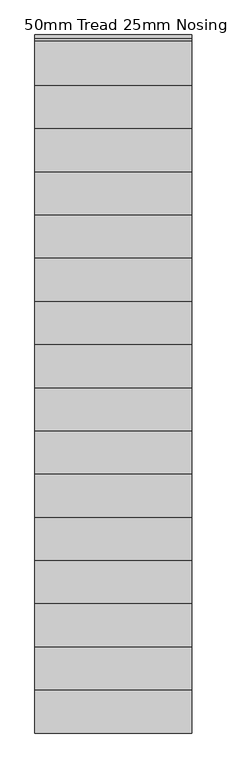
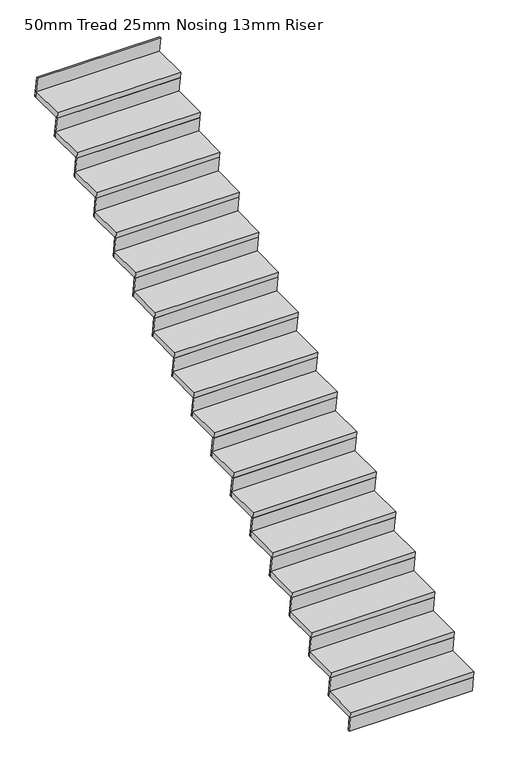
"""IFC4 building model written with IfcOpenShell, lengths in millimetres: stair flight geometry, 50mm Tread 25mm Nosing 13mm Riser."""

from ifc_helpers import new_model, si_unit, frame, origin, place, context, project, spatial, polyline, outline, extrude, source, transform, mapped, element, save


def stair_flight_50mm_tread_25mm_nosing_13mm_riser_8afb8e9e(model_context):
    return source(origin(), model_context, "Body", "SweptSolid", [
        extrude(outline(polyline([(-30533.3785178, 176.4705882), (-30233.3785178, 176.4705882), (-30226.2951845, 126.4705882), (-30526.2951845, 126.4705882), (-30533.3785178, 176.4705882)])), frame((125666.3174172, 0.0, 0.0), z_axis=(1.0, 0.0, 0.0), x_axis=(0.0, 1.0, 0.0)), (0.0, 0.0, 1.0), 1000.0),
        extrude(outline(polyline([(-30526.2951845, 126.4705882), (-30513.6703736, 126.4705882), (-30495.7537069, 0.0), (-30508.3785178, 0.0), (-30526.2951845, 126.4705882)])), frame((125666.3174172, 0.0, 0.0), z_axis=(1.0, 0.0, 0.0), x_axis=(0.0, 1.0, 0.0)), (0.0, 0.0, 1.0), 1000.0),
        extrude(outline(polyline([(-30251.2951845, 302.9411765), (-30238.6703736, 302.9411765), (-30213.6703736, 126.4705882), (-30226.2951845, 126.4705882), (-30251.2951845, 302.9411765)])), frame((125666.3174172, 0.0, 0.0), z_axis=(1.0, 0.0, 0.0), x_axis=(0.0, 1.0, 0.0)), (0.0, 0.0, 1.0), 1000.0),
        extrude(outline(polyline([(-30258.3785178, 352.9411765), (-29958.3785178, 352.9411765), (-29951.2951845, 302.9411765), (-30251.2951845, 302.9411765), (-30258.3785178, 352.9411765)])), frame((125666.3174172, 0.0, 0.0), z_axis=(1.0, 0.0, 0.0), x_axis=(0.0, 1.0, 0.0)), (0.0, 0.0, 1.0), 1000.0),
        extrude(outline(polyline([(-29976.2951845, 479.4117647), (-29963.6703736, 479.4117647), (-29938.6703736, 302.9411765), (-29951.2951845, 302.9411765), (-29976.2951845, 479.4117647)])), frame((125666.3174172, 0.0, 0.0), z_axis=(1.0, 0.0, 0.0), x_axis=(0.0, 1.0, 0.0)), (0.0, 0.0, 1.0), 1000.0),
        extrude(outline(polyline([(-29983.3785178, 529.4117647), (-29683.3785178, 529.4117647), (-29676.2951845, 479.4117647), (-29976.2951845, 479.4117647), (-29983.3785178, 529.4117647)])), frame((125666.3174172, 0.0, 0.0), z_axis=(1.0, 0.0, 0.0), x_axis=(0.0, 1.0, 0.0)), (0.0, 0.0, 1.0), 1000.0),
        extrude(outline(polyline([(-29701.2951845, 655.8823529), (-29688.6703736, 655.8823529), (-29663.6703736, 479.4117647), (-29676.2951845, 479.4117647), (-29701.2951845, 655.8823529)])), frame((125666.3174172, 0.0, 0.0), z_axis=(1.0, 0.0, 0.0), x_axis=(0.0, 1.0, 0.0)), (0.0, 0.0, 1.0), 1000.0),
        extrude(outline(polyline([(-29708.3785178, 705.8823529), (-29408.3785178, 705.8823529), (-29401.2951845, 655.8823529), (-29701.2951845, 655.8823529), (-29708.3785178, 705.8823529)])), frame((125666.3174172, 0.0, 0.0), z_axis=(1.0, 0.0, 0.0), x_axis=(0.0, 1.0, 0.0)), (0.0, 0.0, 1.0), 1000.0),
        extrude(outline(polyline([(-29426.2951845, 832.3529412), (-29413.6703736, 832.3529412), (-29388.6703736, 655.8823529), (-29401.2951845, 655.8823529), (-29426.2951845, 832.3529412)])), frame((125666.3174172, 0.0, 0.0), z_axis=(1.0, 0.0, 0.0), x_axis=(0.0, 1.0, 0.0)), (0.0, 0.0, 1.0), 1000.0),
        extrude(outline(polyline([(-29433.3785178, 882.3529412), (-29133.3785178, 882.3529412), (-29126.2951845, 832.3529412), (-29426.2951845, 832.3529412), (-29433.3785178, 882.3529412)])), frame((125666.3174172, 0.0, 0.0), z_axis=(1.0, 0.0, 0.0), x_axis=(0.0, 1.0, 0.0)), (0.0, 0.0, 1.0), 1000.0),
        extrude(outline(polyline([(-29151.2951845, 1008.8235294), (-29138.6703736, 1008.8235294), (-29113.6703736, 832.3529412), (-29126.2951845, 832.3529412), (-29151.2951845, 1008.8235294)])), frame((125666.3174172, 0.0, 0.0), z_axis=(1.0, 0.0, 0.0), x_axis=(0.0, 1.0, 0.0)), (0.0, 0.0, 1.0), 1000.0),
        extrude(outline(polyline([(-29158.3785178, 1058.8235294), (-28858.3785178, 1058.8235294), (-28851.2951845, 1008.8235294), (-29151.2951845, 1008.8235294), (-29158.3785178, 1058.8235294)])), frame((125666.3174172, 0.0, 0.0), z_axis=(1.0, 0.0, 0.0), x_axis=(0.0, 1.0, 0.0)), (0.0, 0.0, 1.0), 1000.0),
        extrude(outline(polyline([(-28876.2951845, 1185.2941176), (-28863.6703736, 1185.2941176), (-28838.6703736, 1008.8235294), (-28851.2951845, 1008.8235294), (-28876.2951845, 1185.2941176)])), frame((125666.3174172, 0.0, 0.0), z_axis=(1.0, 0.0, 0.0), x_axis=(0.0, 1.0, 0.0)), (0.0, 0.0, 1.0), 1000.0),
        extrude(outline(polyline([(-28883.3785178, 1235.2941176), (-28583.3785178, 1235.2941176), (-28576.2951845, 1185.2941176), (-28876.2951845, 1185.2941176), (-28883.3785178, 1235.2941176)])), frame((125666.3174172, 0.0, 0.0), z_axis=(1.0, 0.0, 0.0), x_axis=(0.0, 1.0, 0.0)), (0.0, 0.0, 1.0), 1000.0),
        extrude(outline(polyline([(-28601.2951845, 1361.7647059), (-28588.6703736, 1361.7647059), (-28563.6703736, 1185.2941176), (-28576.2951845, 1185.2941176), (-28601.2951845, 1361.7647059)])), frame((125666.3174172, 0.0, 0.0), z_axis=(1.0, 0.0, 0.0), x_axis=(0.0, 1.0, 0.0)), (0.0, 0.0, 1.0), 1000.0),
        extrude(outline(polyline([(-28608.3785178, 1411.7647059), (-28308.3785178, 1411.7647059), (-28301.2951845, 1361.7647059), (-28601.2951845, 1361.7647059), (-28608.3785178, 1411.7647059)])), frame((125666.3174172, 0.0, 0.0), z_axis=(1.0, 0.0, 0.0), x_axis=(0.0, 1.0, 0.0)), (0.0, 0.0, 1.0), 1000.0),
        extrude(outline(polyline([(-28326.2951845, 1538.2352941), (-28313.6703736, 1538.2352941), (-28288.6703736, 1361.7647059), (-28301.2951845, 1361.7647059), (-28326.2951845, 1538.2352941)])), frame((125666.3174172, 0.0, 0.0), z_axis=(1.0, 0.0, 0.0), x_axis=(0.0, 1.0, 0.0)), (0.0, 0.0, 1.0), 1000.0),
        extrude(outline(polyline([(-28333.3785178, 1588.2352941), (-28033.3785178, 1588.2352941), (-28026.2951845, 1538.2352941), (-28326.2951845, 1538.2352941), (-28333.3785178, 1588.2352941)])), frame((125666.3174172, 0.0, 0.0), z_axis=(1.0, 0.0, 0.0), x_axis=(0.0, 1.0, 0.0)), (0.0, 0.0, 1.0), 1000.0),
        extrude(outline(polyline([(-28051.2951845, 1714.7058824), (-28038.6703736, 1714.7058824), (-28013.6703736, 1538.2352941), (-28026.2951845, 1538.2352941), (-28051.2951845, 1714.7058824)])), frame((125666.3174172, 0.0, 0.0), z_axis=(1.0, 0.0, 0.0), x_axis=(0.0, 1.0, 0.0)), (0.0, 0.0, 1.0), 1000.0),
        extrude(outline(polyline([(-28058.3785178, 1764.7058824), (-27758.3785178, 1764.7058824), (-27751.2951845, 1714.7058824), (-28051.2951845, 1714.7058824), (-28058.3785178, 1764.7058824)])), frame((125666.3174172, 0.0, 0.0), z_axis=(1.0, 0.0, 0.0), x_axis=(0.0, 1.0, 0.0)), (0.0, 0.0, 1.0), 1000.0),
        extrude(outline(polyline([(-27776.2951845, 1891.1764706), (-27763.6703736, 1891.1764706), (-27738.6703736, 1714.7058824), (-27751.2951845, 1714.7058824), (-27776.2951845, 1891.1764706)])), frame((125666.3174172, 0.0, 0.0), z_axis=(1.0, 0.0, 0.0), x_axis=(0.0, 1.0, 0.0)), (0.0, 0.0, 1.0), 1000.0),
        extrude(outline(polyline([(-27783.3785178, 1941.1764706), (-27483.3785178, 1941.1764706), (-27476.2951845, 1891.1764706), (-27776.2951845, 1891.1764706), (-27783.3785178, 1941.1764706)])), frame((125666.3174172, 0.0, 0.0), z_axis=(1.0, 0.0, 0.0), x_axis=(0.0, 1.0, 0.0)), (0.0, 0.0, 1.0), 1000.0),
        extrude(outline(polyline([(-27501.2951845, 2067.6470588), (-27488.6703736, 2067.6470588), (-27463.6703736, 1891.1764706), (-27476.2951845, 1891.1764706), (-27501.2951845, 2067.6470588)])), frame((125666.3174172, 0.0, 0.0), z_axis=(1.0, 0.0, 0.0), x_axis=(0.0, 1.0, 0.0)), (0.0, 0.0, 1.0), 1000.0),
        extrude(outline(polyline([(-27508.3785178, 2117.6470588), (-27208.3785178, 2117.6470588), (-27201.2951845, 2067.6470588), (-27501.2951845, 2067.6470588), (-27508.3785178, 2117.6470588)])), frame((125666.3174172, 0.0, 0.0), z_axis=(1.0, 0.0, 0.0), x_axis=(0.0, 1.0, 0.0)), (0.0, 0.0, 1.0), 1000.0),
        extrude(outline(polyline([(-27226.2951845, 2244.1176471), (-27213.6703736, 2244.1176471), (-27188.6703736, 2067.6470588), (-27201.2951845, 2067.6470588), (-27226.2951845, 2244.1176471)])), frame((125666.3174172, 0.0, 0.0), z_axis=(1.0, 0.0, 0.0), x_axis=(0.0, 1.0, 0.0)), (0.0, 0.0, 1.0), 1000.0),
        extrude(outline(polyline([(-27233.3785178, 2294.1176471), (-26933.3785178, 2294.1176471), (-26926.2951845, 2244.1176471), (-27226.2951845, 2244.1176471), (-27233.3785178, 2294.1176471)])), frame((125666.3174172, 0.0, 0.0), z_axis=(1.0, 0.0, 0.0), x_axis=(0.0, 1.0, 0.0)), (0.0, 0.0, 1.0), 1000.0),
        extrude(outline(polyline([(-26951.2951845, 2420.5882353), (-26938.6703736, 2420.5882353), (-26913.6703736, 2244.1176471), (-26926.2951845, 2244.1176471), (-26951.2951845, 2420.5882353)])), frame((125666.3174172, 0.0, 0.0), z_axis=(1.0, 0.0, 0.0), x_axis=(0.0, 1.0, 0.0)), (0.0, 0.0, 1.0), 1000.0),
        extrude(outline(polyline([(-26958.3785178, 2470.5882353), (-26658.3785178, 2470.5882353), (-26651.2951845, 2420.5882353), (-26951.2951845, 2420.5882353), (-26958.3785178, 2470.5882353)])), frame((125666.3174172, 0.0, 0.0), z_axis=(1.0, 0.0, 0.0), x_axis=(0.0, 1.0, 0.0)), (0.0, 0.0, 1.0), 1000.0),
        extrude(outline(polyline([(-26676.2951845, 2597.0588235), (-26663.6703736, 2597.0588235), (-26638.6703736, 2420.5882353), (-26651.2951845, 2420.5882353), (-26676.2951845, 2597.0588235)])), frame((125666.3174172, 0.0, 0.0), z_axis=(1.0, 0.0, 0.0), x_axis=(0.0, 1.0, 0.0)), (0.0, 0.0, 1.0), 1000.0),
        extrude(outline(polyline([(-26683.3785178, 2647.0588235), (-26383.3785178, 2647.0588235), (-26376.2951845, 2597.0588235), (-26676.2951845, 2597.0588235), (-26683.3785178, 2647.0588235)])), frame((125666.3174172, 0.0, 0.0), z_axis=(1.0, 0.0, 0.0), x_axis=(0.0, 1.0, 0.0)), (0.0, 0.0, 1.0), 1000.0),
        extrude(outline(polyline([(-26401.2951845, 2773.5294118), (-26388.6703736, 2773.5294118), (-26363.6703736, 2597.0588235), (-26376.2951845, 2597.0588235), (-26401.2951845, 2773.5294118)])), frame((125666.3174172, 0.0, 0.0), z_axis=(1.0, 0.0, 0.0), x_axis=(0.0, 1.0, 0.0)), (0.0, 0.0, 1.0), 1000.0),
        extrude(outline(polyline([(-26126.2951845, 2950.0), (-26113.6703736, 2950.0), (-26088.6703736, 2773.5294118), (-26101.2951845, 2773.5294118), (-26126.2951845, 2950.0)])), frame((125666.3174172, 0.0, 0.0), z_axis=(1.0, 0.0, 0.0), x_axis=(0.0, 1.0, 0.0)), (0.0, 0.0, 1.0), 1000.0),
        extrude(outline(polyline([(-26408.3785178, 2823.5294118), (-26108.3785178, 2823.5294118), (-26101.2951845, 2773.5294118), (-26401.2951845, 2773.5294118), (-26408.3785178, 2823.5294118)])), frame((125666.3174172, 0.0, 0.0), z_axis=(1.0, 0.0, 0.0), x_axis=(0.0, 1.0, 0.0)), (0.0, 0.0, 1.0), 1000.0),
    ])


if __name__ == "__main__":
    model = new_model("IFC4")
    model_context = context("Model", 3, world=origin())
    ifc_project = project(units=[si_unit("LENGTHUNIT", "METRE", prefix="MILLI")], contexts=[model_context])
    site = spatial("IfcSite", under=ifc_project)
    building = spatial("IfcBuilding", under=site)
    placement = place(None, origin())
    stair_flight_50mm_tread_25mm_nosing_13mm_riser_shape = stair_flight_50mm_tread_25mm_nosing_13mm_riser_8afb8e9e(model_context)
    element("IfcStairFlight", 1, ObjectType="50mm Tread 25mm Nosing 13mm Riser", at=placement, inside=building, context=model_context, shape_type="MappedRepresentation", body=[
        mapped(stair_flight_50mm_tread_25mm_nosing_13mm_riser_shape, transform((0.0, 0.0, 0.0), x_axis=(1.0, 0.0, 0.0), y_axis=(0.0, 1.0, 0.0), z_axis=(0.0, 0.0, 1.0))),
    ])
    save(model, "model.ifc")
